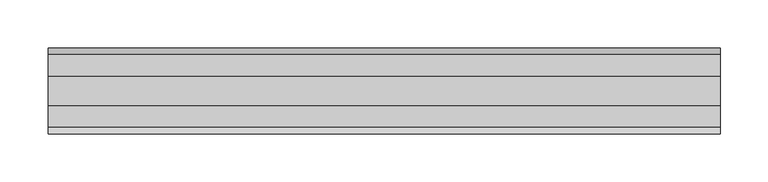
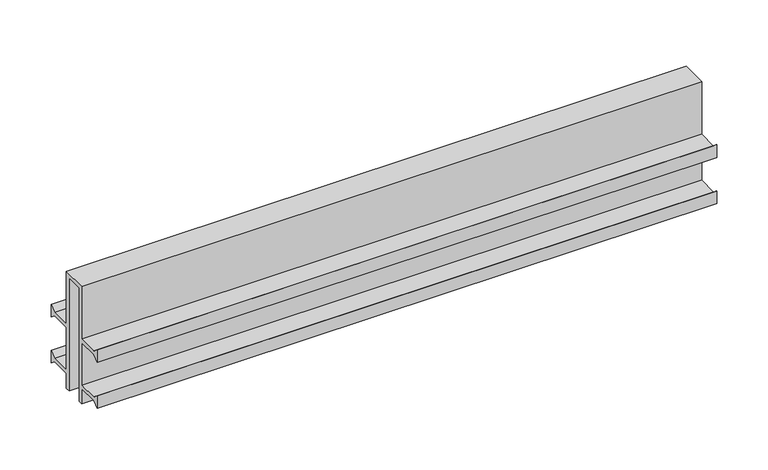
"""IFC4 building model written with IfcOpenShell, lengths in millimetres: proxy geometry, TN_Гидрошпонка ТН Фундамент : Гидрошпонка ТН Фундамент ДШП-В-20."""

from ifc_helpers import new_model, si_unit, frame, origin, place, context, project, spatial, polyline, outline, extrude, source, transform, mapped, element, save


def specialty_equipment_b78296aa(model_context):
    return source(origin(), model_context, "Body", "SweptSolid", [
        extrude(outline(polyline([(10.0, -5.0), (-10.0, -5.0), (-10.0, -140.0), (-15.0, -140.0), (-15.0, -122.1), (-38.120566, -122.1), (-45.0, -127.5), (-45.0, -112.5), (-38.120566, -117.9), (-15.0, -117.9), (-15.0, -67.1), (-38.120566, -67.1), (-45.0, -72.5), (-45.0, -57.5), (-38.120566, -62.9), (-15.0, -62.9), (-15.0, 0.0), (15.0, 0.0), (15.0, -62.9), (38.120566, -62.9), (45.0, -57.5), (45.0, -72.5), (38.120566, -67.1), (15.0, -67.1), (15.0, -117.9), (38.120566, -117.9), (45.0, -112.5), (45.0, -127.5), (38.120566, -122.1), (15.0, -122.1), (15.0, -140.0), (10.0, -140.0), (10.0, -5.0)])), frame((0.0, 0.0, 0.0), z_axis=(1.0, 0.0, 0.0), x_axis=(0.0, 1.0, 0.0)), (0.0, 0.0, 1.0), 700.0),
    ])


if __name__ == "__main__":
    model = new_model("IFC4")
    model_context = context("Model", 3, world=origin())
    ifc_project = project(units=[si_unit("LENGTHUNIT", "METRE", prefix="MILLI")], contexts=[model_context])
    site = spatial("IfcSite", under=ifc_project)
    building = spatial("IfcBuilding", under=site)
    placement = place(None, origin())
    specialty_equipment_shape = specialty_equipment_b78296aa(model_context)
    element("IfcBuildingElementProxy", 1, Name="TN_Гидрошпонка ТН Фундамент : Гидрошпонка ТН Фундамент ДШП-В-20", ObjectType="TN_Гидрошпонка ТН Фундамент : Гидрошпонка ТН Фундамент ДШП-В-20", at=placement, inside=building, context=model_context, shape_type="MappedRepresentation", body=[
        mapped(specialty_equipment_shape, transform((0.0, 0.0, 0.0), x_axis=(1.0, 0.0, 0.0), y_axis=(0.0, 1.0, 0.0), z_axis=(0.0, 0.0, 1.0))),
    ])
    save(model, "model.ifc")

# Revit data of these elements
# Type "TN_Гидрошпонка ТН Фундамент : Гидрошпонка ТН Фундамент ДШП-В-20"
#   Description = "Внутренние П-образные гидроизоляционные шпонки ТН Фундамент ДШП-В представляют собой профилированную ленту, изготовленную из пластифицированного поливинилхлорида методом экструзии."
#   Type Comments = "п.м."
#   Manufacturer = "ТехноНИКОЛЬ"
#   URL = "https://nav.tn.ru/catalog/gidroizolyatsiya/komplektatsiya-dlya-gidroizolyatsii/gidroshponki-tekhnonikol-fundament-dshp-v/"
#   ADSK_Примечание = ""
#   ADSK_Обозначение [instance default] = "ТехноНИКОЛЬ"
#   ADSK_Наименование = "Гидрошпонка ТН Фундамент ДШП-В-20"
#   ADSK_Масса_Текст = ""
#   ADSK_Марка = ""
#   ADSK_Код изделия = "72232"
#   ADSK_Завод-изготовитель [instance default] = "ТехноНИКОЛЬ"
#   ADSK_Единица измерения [instance default] = "п.м."
#   ADSK_Группирование = "Гидрошпонки"
#   ADSK_URL страницы изделия = "https://nav.tn.ru/catalog/gidroizolyatsiya/komplektatsiya-dlya-gidroizolyatsii/gidroshponki-tekhnonikol-fundament-dshp-v/"
#   ADSK_URL документации изделия = "https://nav.tn.ru/upload/iblock/bef/50ps2dij0orvk11owm0y8tn3vby3otsm/Tekhlist-7.405_Gidroshponki_TN_Fundament_DSHP_V_RU_ru.pdf"
#   built-in parameter 1001306 [instance default] = 3.28084 (stored number, unit not read)
#   ADSK_Размер_Длина [instance default] = 1000 mm
#   ADSK_Количество [instance default] = 1
#   Гидрошпонка ТН Фундамент ТШ-Н-210 = no
#   Гидрошпонка ТН Фундамент ДШП-В-50 = no
#   Гидрошпонка ТН Фундамент ДШП-В-20 = yes
#   Гидрошпонка ТН Фундамент ДШ-В-280 = no
#   Гидрошпонка ТН Фундамент ДШ-В-250 = no
#   Гидрошпонка ТН Фундамент ТШ-В-250 = no
#   Гидрошпонка ТН Фундамент ТПС-В 140-1 = no
#   Гидрошпонка ТН Фундамент ДШ-Н-280 = no
#   Гидрошпонка ТН Фундамент ДШ-Н-250 = no
#   Гидрошпонка ТН Фундамент ТПС-В 100-2 = no
#   Гидрошпонка ТН Фундамент ТШ-Н-250 = no
#   Гидрошпонка ТН Фундамент ТШ-В-210 = no
#   Материал = TN_ПВХ_Черный
#   Default Elevation = 0
# Element 1 (IfcBuildingElementProxy, "TN_Гидрошпонка ТН Фундамент : Гидрошпонка ТН Фундамент ДШП-В-20")
#   built-in parameter 1001306 = 2.29659 (stored number, unit not read)
#   ADSK_Размер_Длина = 700 mm
#   ADSK_Количество = 0.7
#   Materials on its faces: "TN_ПВХ_Черный"
# Materials
#   "TN_ПВХ_Черный": class "Типовые", colour RGB 48 48 48, transparency 0, Cost = 0
